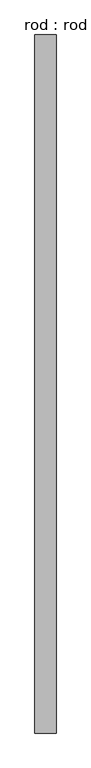
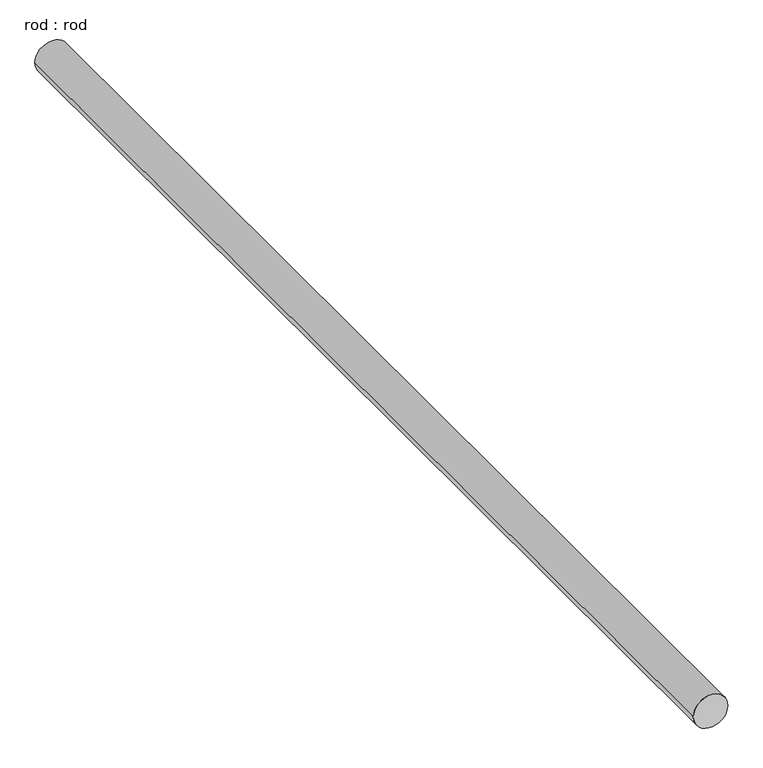
"""IFC4 building model written with IfcOpenShell, lengths in millimetres: proxy geometry, rod : rod."""

from ifc_helpers import new_model, si_unit, point, frame, frame_2d, origin, place, context, project, spatial, circle_curve, trimmed, segment, composite_curve, outline, extrude, source, transform, mapped, element, save


def rod_rod_79d3e298(model_context):
    return source(origin(), model_context, "Body", "SweptSolid", [
        extrude(outline(composite_curve([segment(trimmed(circle_curve(frame_2d((0.0108462, 0.0)), 200.0), [point((0.0108462, 200.0))], [point((0.0108462, -200.0))], False, "CARTESIAN"), True, "CONTINUOUS"), segment(trimmed(circle_curve(frame_2d((0.0108462, 0.0)), 200.0), [point((0.0108462, -200.0))], [point((0.0108462, 200.0))], False, "CARTESIAN"), True, "CONTINUOUS")], self_intersect=False)), frame((0.0, -2525.8092515, 0.0), z_axis=(0.0, 1.0, 0.0), x_axis=(0.0, 0.0, 1.0)), (0.0, 0.0, 1.0), 13237.0757337),
    ])


if __name__ == "__main__":
    model = new_model("IFC4")
    model_context = context("Model", 3, world=origin())
    ifc_project = project(units=[si_unit("LENGTHUNIT", "METRE", prefix="MILLI")], contexts=[model_context])
    site = spatial("IfcSite", under=ifc_project)
    building = spatial("IfcBuilding", under=site)
    placement = place(None, origin())
    rod_rod_shape = rod_rod_79d3e298(model_context)
    element("IfcBuildingElementProxy", 1, Name="rod : rod", ObjectType="rod : rod", at=placement, inside=building, context=model_context, shape_type="MappedRepresentation", body=[
        mapped(rod_rod_shape, transform((0.0, 0.0, 0.0), x_axis=(1.0, 0.0, 0.0), y_axis=(0.0, 1.0, 0.0), z_axis=(0.0, 0.0, 1.0))),
    ])
    save(model, "model.ifc")

# Revit data of these elements
# Type "rod : rod"
#   Default Elevation = 0
